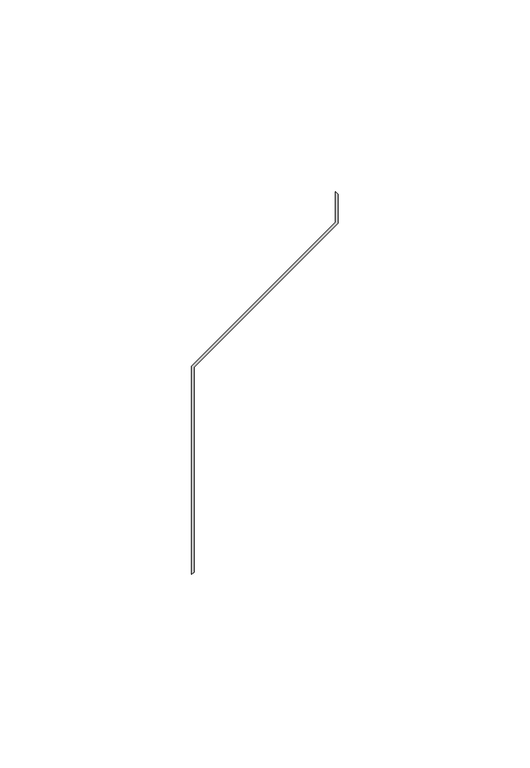
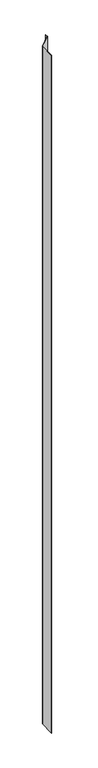
"""IFC4 building model written with IfcOpenShell, lengths in millimetres: proxy geometry, MBCI 7.2-V Panel4 : MBCI 7.2-V Panel-1."""

import ifcopenshell
import ifcopenshell.guid

model = None  # the IFC model being written
_history = None  # IfcOwnerHistory: only IFC2X3 demands one
_inside = {}  # id of a spatial element -> (the spatial element, [elements in it])
_under = {}  # id of a project, library or spatial element -> (it, [spatial elements below it])
_declared = {}  # id of a project -> (the project, [libraries it declares])
_typed = {}  # id of a type object -> (the type object, [elements of that type])
_made_of = {}  # id of a material, layer set ... -> (it, [elements and type objects made of it])


def new_model(schema):
    """Start an empty IFC model of exactly this schema.

    Asked for "IFC4X3", IfcOpenShell would pick the latest addendum, in which some entities
    have other attributes; the version numbers below select the first issue.
    IFC2X3 requires an IfcOwnerHistory on every rooted entity: one is made here for all.
    """
    global model, _history
    if schema == "IFC4X3":
        model = ifcopenshell.file(schema_version=(4, 3, 0, 0))
    else:
        model = ifcopenshell.file(schema=schema)
    _inside.clear()
    _under.clear()
    _declared.clear()
    _typed.clear()
    _made_of.clear()
    _history = None
    if model.schema == "IFC2X3":
        org = make("IfcOrganization", Name="unknown")
        user = make(
            "IfcPersonAndOrganization",
            ThePerson=make("IfcPerson", FamilyName="unknown"),
            TheOrganization=org,
        )
        app = make(
            "IfcApplication",
            ApplicationDeveloper=org,
            Version="unknown",
            ApplicationFullName="unknown",
            ApplicationIdentifier="unknown",
        )
        _history = make(
            "IfcOwnerHistory",
            OwningUser=user,
            OwningApplication=app,
            ChangeAction="ADDED",
            CreationDate=0,
        )
    return model


def make(cls, **values):
    """One entity of the class cls with the attributes given. An attribute that is None is left unset."""
    return model.create_entity(
        cls, **{name: value for name, value in values.items() if value is not None}
    )


def rooted(cls, **values):
    """An entity with a GlobalId (a new one), such as an element, a storey or a relation."""
    return make(cls, GlobalId=ifcopenshell.guid.new(), OwnerHistory=_history, **values)


def si_unit(unit_type, name, prefix=None):
    """IfcSIUnit, for example si_unit("LENGTHUNIT", "METRE", prefix="MILLI")."""
    return make("IfcSIUnit", UnitType=unit_type, Prefix=prefix, Name=name)


def assignment(units):
    """IfcUnitAssignment: the units of a project."""
    return None if units is None else make("IfcUnitAssignment", Units=units)


def point(xyz):
    """IfcCartesianPoint."""
    return None if xyz is None else make("IfcCartesianPoint", Coordinates=xyz)


def direction(xyz):
    """IfcDirection."""
    return None if xyz is None else make("IfcDirection", DirectionRatios=xyz)


def frame(location, z_axis=None, x_axis=None):
    """IfcAxis2Placement3D, a coordinate frame: its origin and axes. An axis left out is left unset."""
    return make(
        "IfcAxis2Placement3D",
        Location=point(location),
        Axis=direction(z_axis),
        RefDirection=direction(x_axis),
    )


def origin():
    """The frame at (0, 0, 0) with its axes left unset."""
    return frame((0.0, 0.0, 0.0))


def place(relative_to, where):
    """IfcLocalPlacement: puts the frame where relative to a parent placement (None: the world)."""
    return make(
        "IfcLocalPlacement", PlacementRelTo=relative_to, RelativePlacement=where
    )


def context(
    kind, dimensions, precision=None, world=None, true_north=None, identifier=None
):
    """IfcGeometricRepresentationContext, for example the 3D "Model" context."""
    return make(
        "IfcGeometricRepresentationContext",
        ContextIdentifier=identifier,
        ContextType=kind,
        CoordinateSpaceDimension=dimensions,
        Precision=precision,
        WorldCoordinateSystem=world,
        TrueNorth=true_north,
    )


def project(units=None, contexts=None):
    """IfcProject with its units and contexts."""
    return rooted(
        "IfcProject",
        Name="project",
        RepresentationContexts=contexts,
        UnitsInContext=assignment(units),
    )


def spatial(cls, under=None, at=None, **own):
    """A site, building, storey or space (cls), placed at a placement, below another one or the project."""
    s = rooted(cls, ObjectPlacement=at, **own)
    if under is not None:
        _under.setdefault(under.id(), (under, []))[1].append(s)
    return s


def polyline(points):
    """IfcPolyline through the points."""
    return make("IfcPolyline", Points=[point(p) for p in points])


def outline(outer, holes=None, kind="AREA"):
    """IfcArbitraryClosedProfileDef: a profile drawn as a closed curve; with holes, ...WithVoids."""
    if holes is None:
        return make("IfcArbitraryClosedProfileDef", ProfileType=kind, OuterCurve=outer)
    return make(
        "IfcArbitraryProfileDefWithVoids",
        ProfileType=kind,
        OuterCurve=outer,
        InnerCurves=holes,
    )


def extrude(swept, where, along, depth):
    """IfcExtrudedAreaSolid: the profile swept, set in the frame where, extruded along a direction by depth."""
    return make(
        "IfcExtrudedAreaSolid",
        SweptArea=swept,
        Position=where,
        ExtrudedDirection=direction(along),
        Depth=depth,
    )


def shape(context_of_items, identifier, shape_type, items):
    """IfcShapeRepresentation: the items that make up one representation, for example the "Body"."""
    return make(
        "IfcShapeRepresentation",
        ContextOfItems=context_of_items,
        RepresentationIdentifier=identifier,
        RepresentationType=shape_type,
        Items=items,
    )


def source(mapping_origin, context_of_items, identifier, shape_type, items):
    """IfcRepresentationMap: a shape defined once, which mapped items show again and again."""
    return make(
        "IfcRepresentationMap",
        MappingOrigin=mapping_origin,
        MappedRepresentation=shape(context_of_items, identifier, shape_type, items),
    )


def transform(
    local_origin,
    x_axis=None,
    y_axis=None,
    z_axis=None,
    scale=None,
    scale2=None,
    scale3=None,
    uniform=True,
):
    """IfcCartesianTransformationOperator3D, or its non-uniform kind. x_axis, y_axis, z_axis: its Axis1, 2, 3."""
    if uniform:
        return make(
            "IfcCartesianTransformationOperator3D",
            Axis1=direction(x_axis),
            Axis2=direction(y_axis),
            LocalOrigin=point(local_origin),
            Scale=scale,
            Axis3=direction(z_axis),
        )
    return make(
        "IfcCartesianTransformationOperator3DnonUniform",
        Axis1=direction(x_axis),
        Axis2=direction(y_axis),
        LocalOrigin=point(local_origin),
        Scale=scale,
        Axis3=direction(z_axis),
        Scale2=scale2,
        Scale3=scale3,
    )


def mapped(mapping_source, mapping_target):
    """IfcMappedItem: shows the shape of a source again, moved by a transform."""
    return make(
        "IfcMappedItem", MappingSource=mapping_source, MappingTarget=mapping_target
    )


def made_of(thing, what):
    """Note that an element or type object is made of a material, layer set ...; save() writes the relation."""
    if what is not None:
        _made_of.setdefault(what.id(), (what, []))[1].append(thing)
    return thing


def element(
    cls,
    number,
    at=None,
    inside=None,
    cuts=None,
    type_object=None,
    material=None,
    context=None,
    identifier="Body",
    shape_type=None,
    held_by="IfcProductDefinitionShape",
    body=None,
    shapes=None,
    **own,
):
    """One element of the class cls, such as IfcWall. Its Tag is "e" and its number.

    at: its placement. inside: the storey or other place that contains it. cuts: it is an
    opening in that element (IfcRelVoidsElement). A single representation is given by context,
    identifier, shape_type and body (its items); several are given by shapes. held_by: the class
    of the entity that holds the representations. save() writes the other relations.
    """
    e = rooted(cls, Tag="e%d" % number, ObjectPlacement=at, **own)
    if body is not None:
        shapes = [shape(context, identifier, shape_type, body)]
    if shapes is not None:
        e.Representation = make(held_by, Representations=shapes)
    if inside is not None:
        _inside.setdefault(inside.id(), (inside, []))[1].append(e)
    if cuts is not None:
        rooted(
            "IfcRelVoidsElement", RelatingBuildingElement=cuts, RelatedOpeningElement=e
        )
    if type_object is not None:
        _typed.setdefault(type_object.id(), (type_object, []))[1].append(e)
    return made_of(e, material)


def aggregate(whole, parts):
    """IfcRelAggregates: a whole, such as a stair, and the parts it consists of."""
    return rooted("IfcRelAggregates", RelatingObject=whole, RelatedObjects=parts)


def save(model, path):
    """Write the relations noted so far, then the file.

    IfcRelAggregates (storeys below a building ...), IfcRelContainedInSpatialStructure (elements
    in a storey), IfcRelDefinesByType, IfcRelAssociatesMaterial and IfcRelDeclares: one each for
    every whole, place, type object, material and project.
    """
    for whole, parts in _under.values():
        aggregate(whole, parts)
    for where, things in _inside.values():
        rooted(
            "IfcRelContainedInSpatialStructure",
            RelatedElements=things,
            RelatingStructure=where,
        )
    for kind, things in _typed.values():
        rooted("IfcRelDefinesByType", RelatedObjects=things, RelatingType=kind)
    for what, things in _made_of.values():
        rooted("IfcRelAssociatesMaterial", RelatedObjects=things, RelatingMaterial=what)
    for by, libraries in _declared.values():
        rooted("IfcRelDeclares", RelatingContext=by, RelatedDefinitions=libraries)
    model.write(path)


def generic_models_61abd2db(model_context):
    return source(origin(), model_context, "Body", "SweptSolid", [
        extrude(outline(polyline([(587328.4903864, -536352.8639068), (587328.4903864, -536406.3026716), (587327.8950739, -536406.8979841), (587327.8950739, -536352.6173202), (587365.3854739, -536315.1269202), (587365.3854739, -536307.2537841), (587365.9807864, -536307.8490966), (587365.9807864, -536315.3735068), (587328.4903864, -536352.8639068)])), frame((0.0, 0.0, 12.7), z_axis=(0.0, 0.0, 1.0), x_axis=(1.0, 0.0, 0.0)), (0.0, 0.0, 1.0), 2425.7),
    ])


if __name__ == "__main__":
    model = new_model("IFC4")
    model_context = context("Model", 3, world=origin())
    ifc_project = project(units=[si_unit("LENGTHUNIT", "METRE", prefix="MILLI")], contexts=[model_context])
    site = spatial("IfcSite", under=ifc_project)
    building = spatial("IfcBuilding", under=site)
    placement = place(None, origin())
    generic_models_shape = generic_models_61abd2db(model_context)
    element("IfcBuildingElementProxy", 1, Name="MBCI 7.2-V Panel4 : MBCI 7.2-V Panel-1", ObjectType="MBCI 7.2-V Panel4 : MBCI 7.2-V Panel-1", at=placement, inside=building, context=model_context, shape_type="MappedRepresentation", body=[
        mapped(generic_models_shape, transform((0.0, 0.0, 0.0), x_axis=(1.0, 0.0, 0.0), y_axis=(0.0, 1.0, 0.0), z_axis=(0.0, 0.0, 1.0))),
    ])
    save(model, "model.ifc")

# Revit data of these elements
# Element 1 (IfcBuildingElementProxy, "MBCI 7.2-V Panel4 : MBCI 7.2-V Panel-1")
#   Materials on its faces: "MTL PANEL"
# Materials
#   "MTL PANEL": class "Generic", colour RGB 239 242 240, transparency 0, Cost = 0
